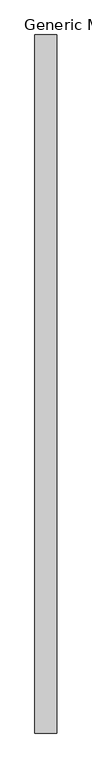
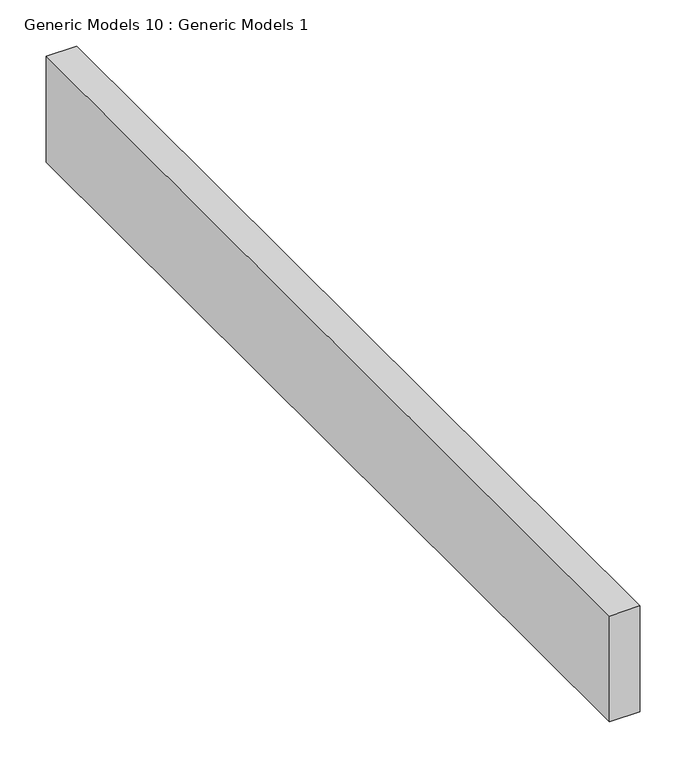
"""IFC4 building model written with IfcOpenShell, lengths in millimetres: proxy geometry, Generic Models 10 : Generic Models 1."""

from ifc_helpers import new_model, si_unit, frame, origin, place, context, project, spatial, polyline, outline, extrude, source, transform, mapped, element, save


def generic_models_10_generic_models_1_ea081297(model_context):
    return source(origin(), model_context, "Body", "SweptSolid", [
        extrude(outline(polyline([(49758.6, 0.0), (49720.5, 0.0), (49720.5, 1219.2), (49758.6, 1219.2), (49758.6, 0.0)])), frame((0.0, 0.0, 5507.83125), z_axis=(0.0, 0.0, 1.0), x_axis=(1.0, 0.0, 0.0)), (0.0, 0.0, 1.0), 139.7),
    ])


if __name__ == "__main__":
    model = new_model("IFC4")
    model_context = context("Model", 3, world=origin())
    ifc_project = project(units=[si_unit("LENGTHUNIT", "METRE", prefix="MILLI")], contexts=[model_context])
    site = spatial("IfcSite", under=ifc_project)
    building = spatial("IfcBuilding", under=site)
    placement = place(None, origin())
    generic_models_10_generic_models_1_shape = generic_models_10_generic_models_1_ea081297(model_context)
    element("IfcBuildingElementProxy", 1, Name="Generic Models 10 : Generic Models 1", ObjectType="Generic Models 10 : Generic Models 1", at=placement, inside=building, context=model_context, shape_type="MappedRepresentation", body=[
        mapped(generic_models_10_generic_models_1_shape, transform((0.0, 0.0, 0.0), x_axis=(1.0, 0.0, 0.0), y_axis=(0.0, 1.0, 0.0), z_axis=(0.0, 0.0, 1.0))),
    ])
    save(model, "model.ifc")

# Revit data of these elements
# Element 1 (IfcBuildingElementProxy, "Generic Models 10 : Generic Models 1")
#   Materials on its faces: "2X BLOCKING - LOCATED AT GRAB BARS, WALL HUNG CABINETS, ETC.)"
# Materials
#   "2X BLOCKING - LOCATED AT GRAB BARS, WALL HUNG CABINETS, ETC.)": class "Wood", colour RGB 234 198 147, transparency 0, Description = "Pinus Echinata", Cost = 0
